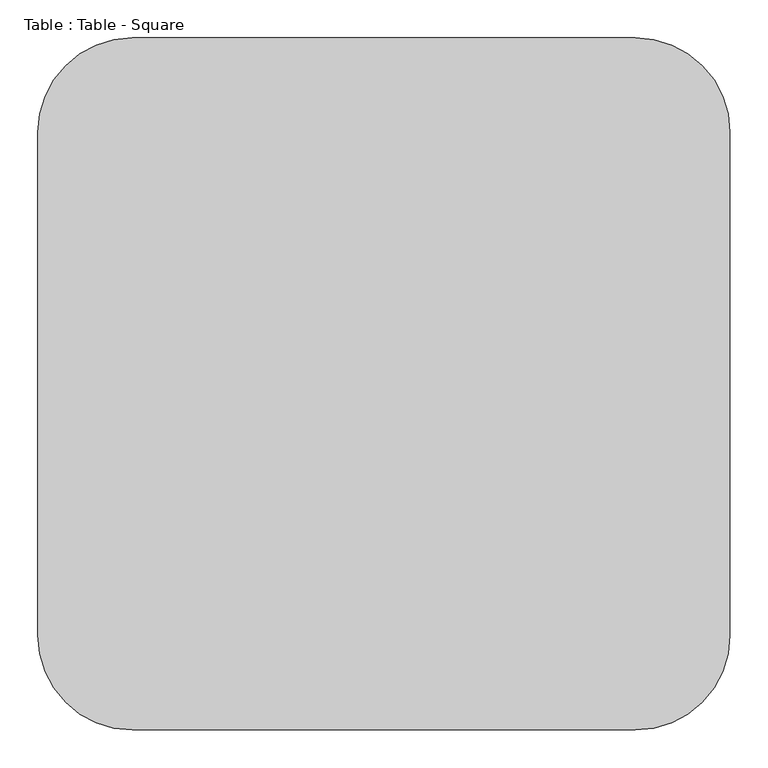
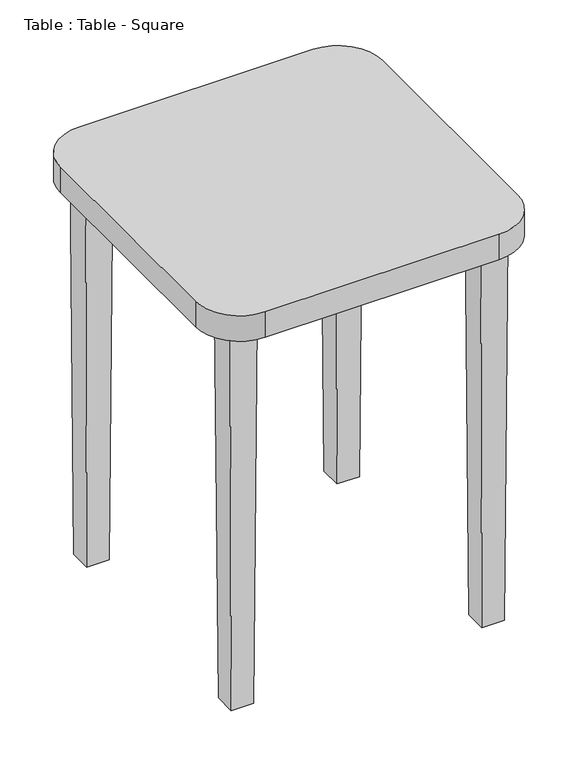
"""IFC4 building model written with IfcOpenShell, lengths in millimetres: proxy geometry, Table : Table - Square."""

from ifc_helpers import new_model, si_unit, point, frame, frame_2d, origin, place, context, project, spatial, polyline, circle_curve, trimmed, segment, composite_curve, outline, extrude, faceted_brep, source, transform, mapped, element, save


def table_table_square_91accc4b(model_context):
    return source(origin(), model_context, "Body", "SolidModel", [
        faceted_brep([(-317.5, -317.5, 1143.0), (-393.7, -317.5, 1143.0), (-393.7, -393.7, 1143.0), (-317.5, -393.7, 1143.0), (-323.85, -323.85, 0.0), (-323.85, -387.35, 0.0), (-387.35, -387.35, 0.0), (-387.35, -323.85, 0.0)], [[[0, 1, 2, 3]], [[4, 5, 6, 7]], [[4, 7, 1, 0]], [[7, 6, 2, 1]], [[6, 5, 3, 2]], [[5, 4, 0, 3]]]),
        faceted_brep([(393.7, -317.5, 1143.0), (317.5, -317.5, 1143.0), (317.5, -393.7, 1143.0), (393.7, -393.7, 1143.0), (387.35, -323.85, 0.0), (387.35, -387.35, 0.0), (323.85, -387.35, 0.0), (323.85, -323.85, 0.0)], [[[0, 1, 2, 3]], [[4, 5, 6, 7]], [[4, 7, 1, 0]], [[7, 6, 2, 1]], [[6, 5, 3, 2]], [[5, 4, 0, 3]]]),
        faceted_brep([(393.7, 393.7, 1143.0), (317.5, 393.7, 1143.0), (317.5, 317.5, 1143.0), (393.7, 317.5, 1143.0), (387.35, 387.35, 0.0), (387.35, 323.85, 0.0), (323.85, 323.85, 0.0), (323.85, 387.35, 0.0)], [[[0, 1, 2, 3]], [[4, 5, 6, 7]], [[4, 7, 1, 0]], [[7, 6, 2, 1]], [[6, 5, 3, 2]], [[5, 4, 0, 3]]]),
        faceted_brep([(-317.5, 393.7, 1143.0), (-393.7, 393.7, 1143.0), (-393.7, 317.5, 1143.0), (-317.5, 317.5, 1143.0), (-323.85, 387.35, 0.0), (-323.85, 323.85, 0.0), (-387.35, 323.85, 0.0), (-387.35, 387.35, 0.0)], [[[0, 1, 2, 3]], [[4, 5, 6, 7]], [[4, 7, 1, 0]], [[7, 6, 2, 1]], [[6, 5, 3, 2]], [[5, 4, 0, 3]]]),
        extrude(outline(composite_curve([segment(trimmed(circle_curve(frame_2d((332.232, 332.232)), 124.968), [point((332.232, 457.2))], [point((457.2, 332.232))], False, "CARTESIAN"), True, "CONTINUOUS"), segment(polyline([(457.2, 332.232), (457.2, -332.232)]), True, "CONTINUOUS"), segment(trimmed(circle_curve(frame_2d((332.232, -332.232)), 124.968), [point((457.2, -332.232))], [point((332.232, -457.2))], False, "CARTESIAN"), True, "CONTINUOUS"), segment(polyline([(332.232, -457.2), (-332.232, -457.2)]), True, "CONTINUOUS"), segment(trimmed(circle_curve(frame_2d((-332.232, -332.232)), 124.968), [point((-332.232, -457.2))], [point((-457.2, -332.232))], False, "CARTESIAN"), True, "CONTINUOUS"), segment(polyline([(-457.2, -332.232), (-457.2, 332.232)]), True, "CONTINUOUS"), segment(trimmed(circle_curve(frame_2d((-332.232, 332.232)), 124.968), [point((-457.2, 332.232))], [point((-332.232, 457.2))], False, "CARTESIAN"), True, "CONTINUOUS"), segment(polyline([(-332.232, 457.2), (332.232, 457.2)]), True, "CONTINUOUS")], self_intersect=False)), frame((0.0, 0.0, 1143.0), z_axis=(0.0, 0.0, 1.0), x_axis=(1.0, 0.0, 0.0)), (0.0, 0.0, 1.0), 76.2),
    ])


if __name__ == "__main__":
    model = new_model("IFC4")
    model_context = context("Model", 3, world=origin())
    ifc_project = project(units=[si_unit("LENGTHUNIT", "METRE", prefix="MILLI")], contexts=[model_context])
    site = spatial("IfcSite", under=ifc_project)
    building = spatial("IfcBuilding", under=site)
    placement = place(None, origin())
    table_table_square_shape = table_table_square_91accc4b(model_context)
    element("IfcBuildingElementProxy", 1, Name="Table : Table - Square", ObjectType="Table : Table - Square", at=placement, inside=building, context=model_context, shape_type="MappedRepresentation", body=[
        mapped(table_table_square_shape, transform((0.0, 0.0, 0.0), x_axis=(1.0, 0.0, 0.0), y_axis=(0.0, 1.0, 0.0), z_axis=(0.0, 0.0, 1.0))),
    ])
    save(model, "model.ifc")

# Revit data of these elements
# Type "Table : Table - Square"
#   Thickness [instance default] = 0' - 2"
#   Sides [instance default] = 3' - 0"
#   Leg Inset [instance default] = 0' - 4"
#   Leg Height [instance default] = 5' - 8"
#   Height [instance default] = 5' - 10"
#   Corner Fillet [instance default] = 0' - 4"
#   Default Elevation = 0
# Element 1 (IfcBuildingElementProxy, "Table : Table - Square")
#   Thickness = 0' - 3"
#   Leg Height = 3' - 9"
#   Height = 4' - 0"
#   Corner Fillet = 0' - 4.92"
